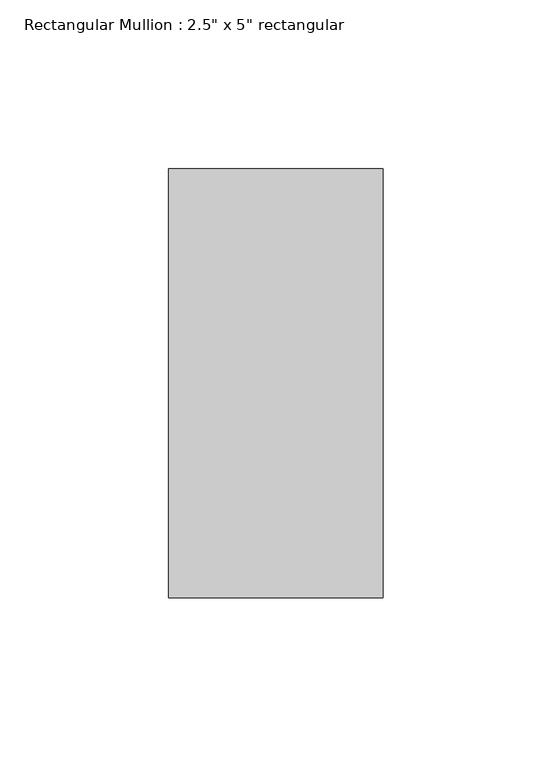
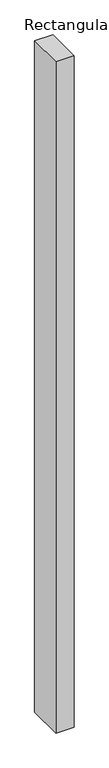
"""IFC4 building model written with IfcOpenShell, lengths in millimetres: member geometry."""

from ifc_helpers import new_model, si_unit, frame, origin, place, context, project, spatial, polyline, outline, extrude, source, transform, mapped, element, save


def member_da42f391(model_context):
    return source(origin(), model_context, "Body", "SweptSolid", [
        extrude(outline(polyline([(31.75, 63.5), (31.75, -63.5), (-31.75, -63.5), (-31.75, 63.5), (31.75, 63.5)])), frame((0.0, 0.0, -2461.8630718), z_axis=(0.0, 0.0, 1.0), x_axis=(1.0, 0.0, 0.0)), (0.0, 0.0, 1.0), 2461.8630718),
    ])


if __name__ == "__main__":
    model = new_model("IFC4")
    model_context = context("Model", 3, world=origin())
    ifc_project = project(units=[si_unit("LENGTHUNIT", "METRE", prefix="MILLI")], contexts=[model_context])
    site = spatial("IfcSite", under=ifc_project)
    building = spatial("IfcBuilding", under=site)
    placement = place(None, origin())
    member_shape = member_da42f391(model_context)
    element("IfcMember", 1, ObjectType="Rectangular Mullion : 2.5\" x 5\" rectangular", at=placement, inside=building, context=model_context, shape_type="MappedRepresentation", body=[
        mapped(member_shape, transform((0.0, 0.0, 0.0), x_axis=(1.0, 0.0, 0.0), y_axis=(0.0, 1.0, 0.0), z_axis=(0.0, 0.0, 1.0))),
    ])
    save(model, "model.ifc")

# Revit data of these elements
# Type "Rectangular Mullion : 2.5\" x 5\" rectangular"
#   built-in parameter 1007304 = 0.416667 (stored number, unit not read)
#   built-in parameter 1007301 = 0.104167 (stored number, unit not read)
#   built-in parameter 1007300 = 0.104167 (stored number, unit not read)
# Element 1 (IfcMember, "Rectangular Mullion : 2.5\" x 5\" rectangular")
#   Materials on its faces: "Aluminum"
# Materials
#   "Aluminum": class "Metal", colour RGB 247 247 247, transparency 0, Description = "Aluminum 6061", Cost = 0
